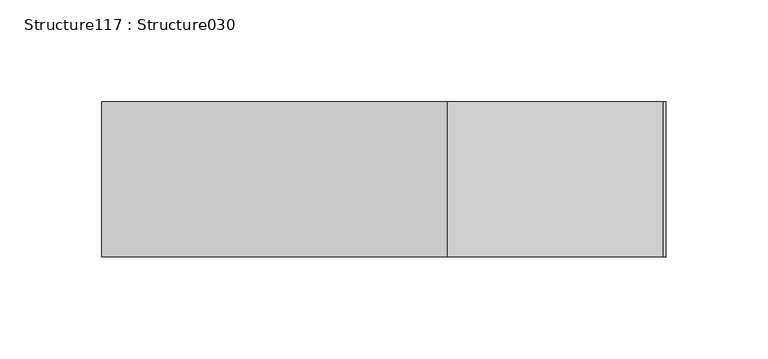
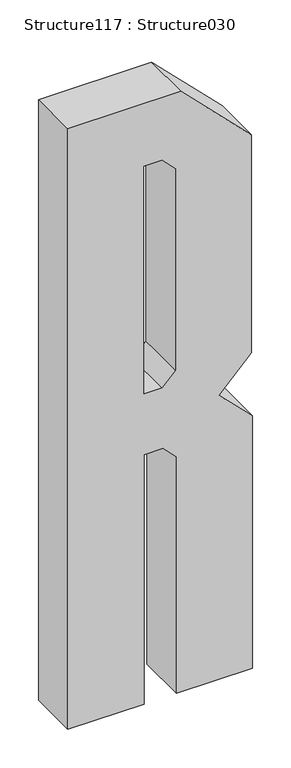
"""IFC4 building model written with IfcOpenShell, lengths in millimetres: proxy geometry, Structure117 : Structure030."""

from ifc_helpers import new_model, si_unit, frame, origin, place, context, project, spatial, polyline, outline, extrude, source, transform, mapped, element, save


def structure117_structure030_9736d06d(model_context):
    return source(origin(), model_context, "Body", "SweptSolid", [
        extrude(outline(polyline([(4374.3842509, -47072.2655751), (4480.4419946, -47178.3233189), (4480.4419946, -47348.2954596), (3528.5825142, -47348.2954596), (3528.5825142, -47234.0857741), (3924.2892507, -47234.0857741), (3924.2892507, -47205.5262677), (3903.8911328, -47185.1281497), (3528.5825142, -47185.1281497), (3528.5825142, -47070.8926431), (3928.3570344, -47070.8926431), (3978.6781441, -47121.2137528), (4028.9992538, -47072.2655751), (4374.3842509, -47072.2655751)]), holes=[polyline([(4020.827159, -47234.0857741), (4381.1897115, -47234.0857741), (4381.1897115, -47206.8821956), (4360.7915935, -47186.4840776), (4041.2277961, -47186.4840776), (4020.827159, -47206.8847147), (4020.827159, -47234.0857741)])]), frame((0.0, 247945.1599557, 0.0), z_axis=(0.0, 1.0, 0.0), x_axis=(0.0, 0.0, 1.0)), (0.0, 0.0, 1.0), 76.2),
    ])


if __name__ == "__main__":
    model = new_model("IFC4")
    model_context = context("Model", 3, world=origin())
    ifc_project = project(units=[si_unit("LENGTHUNIT", "METRE", prefix="MILLI")], contexts=[model_context])
    site = spatial("IfcSite", under=ifc_project)
    building = spatial("IfcBuilding", under=site)
    placement = place(None, origin())
    structure117_structure030_shape = structure117_structure030_9736d06d(model_context)
    element("IfcBuildingElementProxy", 1, Name="Structure117 : Structure030", ObjectType="Structure117 : Structure030", at=placement, inside=building, context=model_context, shape_type="MappedRepresentation", body=[
        mapped(structure117_structure030_shape, transform((0.0, 0.0, 0.0), x_axis=(1.0, 0.0, 0.0), y_axis=(0.0, 1.0, 0.0), z_axis=(0.0, 0.0, 1.0))),
    ])
    save(model, "model.ifc")

# Revit data of these elements
# Type "Structure117 : Structure030"
#   NameOverride = "Structure030"
# Element 1 (IfcBuildingElementProxy, "Structure117 : Structure030")
#   Materials on its faces: "BRUSHED ALUM. LETTERING"
# Materials
#   "BRUSHED ALUM. LETTERING": class "Unassigned", colour RGB 169 181 186, transparency 0, Cost = 0
